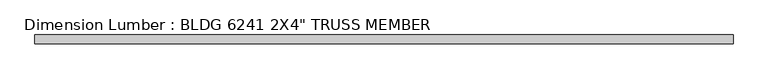
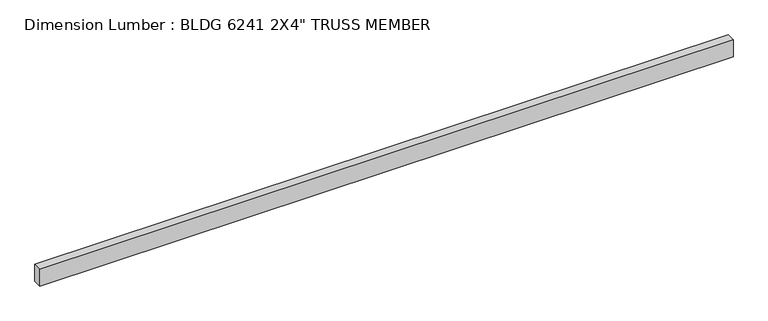
"""IFC4 building model written with IfcOpenShell, lengths in millimetres: beam geometry."""

from ifc_helpers import new_model, si_unit, frame, origin, place, context, project, spatial, polyline, outline, extrude, source, transform, mapped, element, save


def beam_6ddf0adc(model_context):
    return source(origin(), model_context, "Body", "SweptSolid", [
        extrude(outline(polyline([(2020.4829504, 25.4), (2020.4829504, -25.4), (-1995.082951, -25.4), (-1995.082951, 25.4), (2020.4829504, 25.4)])), frame((0.0, 0.0, -50.8), z_axis=(0.0, 0.0, 1.0), x_axis=(1.0, 0.0, 0.0)), (0.0, 0.0, 1.0), 101.6),
    ])


if __name__ == "__main__":
    model = new_model("IFC4")
    model_context = context("Model", 3, world=origin())
    ifc_project = project(units=[si_unit("LENGTHUNIT", "METRE", prefix="MILLI")], contexts=[model_context])
    site = spatial("IfcSite", under=ifc_project)
    building = spatial("IfcBuilding", under=site)
    placement = place(None, origin())
    beam_shape = beam_6ddf0adc(model_context)
    element("IfcBeam", 1, ObjectType="Dimension Lumber : BLDG 6241 2X4\" TRUSS MEMBER", at=placement, inside=building, context=model_context, shape_type="MappedRepresentation", body=[
        mapped(beam_shape, transform((0.0, 0.0, 0.0), x_axis=(1.0, 0.0, 0.0), y_axis=(0.0, 1.0, 0.0), z_axis=(0.0, 0.0, 1.0))),
    ])
    save(model, "model.ifc")

# Revit data of these elements
# Type "Dimension Lumber : BLDG 6241 2X4\" TRUSS MEMBER"
#   Assembly Code = "B10"
#   A = 0.273472 SF
#   Length [instance default] = 5' - 0"
#   b = 0' - 2"
#   d = 0' - 4"
#   Structural Material [instance default] = Softwood, Lumber
# Element 1 (IfcBeam, "Dimension Lumber : BLDG 6241 2X4\" TRUSS MEMBER")
#   Materials on its faces: "Softwood, Lumber"
# Materials
#   "Softwood, Lumber": class "Wood", colour RGB 223 192 134, transparency 0, Description = "Pinus Echinata", Cost = 0
